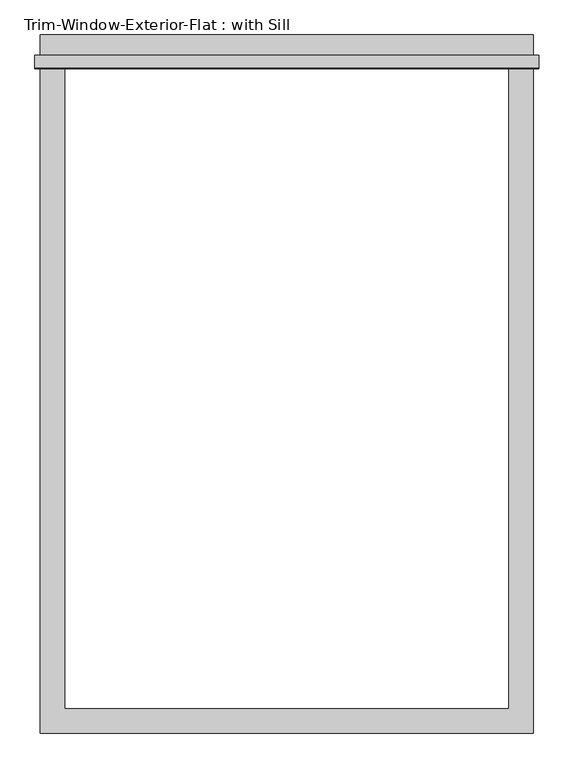
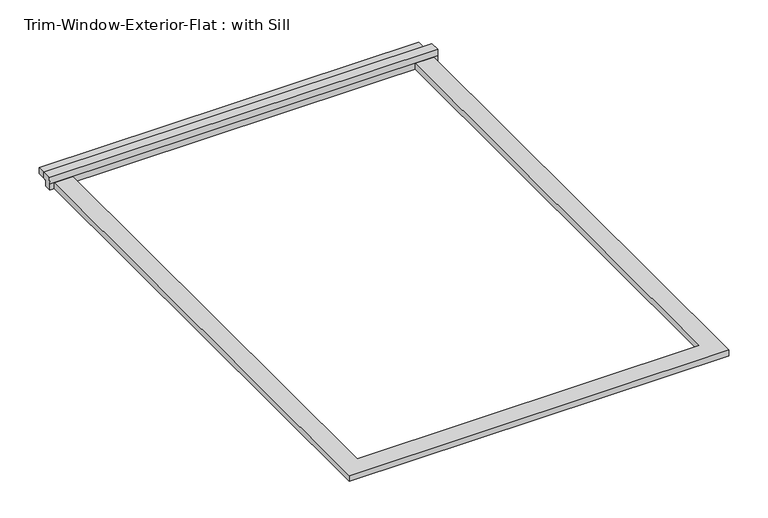
"""IFC4 building model written with IfcOpenShell, lengths in millimetres: proxy geometry, Trim-Window-Exterior-Flat : with Sill."""

from ifc_helpers import new_model, si_unit, frame, origin, origin_with_axes, place, context, project, spatial, polyline, outline, extrude, source, transform, mapped, element, save


def trim_window_exterior_flat_with_sill_a73e42ff(model_context):
    return source(origin(), model_context, "Body", "SweptSolid", [
        extrude(outline(polyline([(577.85, 1520.7823709), (-577.85, 1520.7823709), (-577.85, 1577.9323709), (577.85, 1577.9323709), (577.85, 1520.7823709)])), origin_with_axes(), (0.0, 0.0, 1.0), 19.05),
        extrude(outline(polyline([(1530.35, 38.1), (1530.35, 19.05), (1520.7823709, 19.05), (1520.7823709, 0.0), (1498.6, 0.0), (1498.6, 19.05), (1501.0580645, 38.1), (1530.35, 38.1)])), frame((-590.55, 0.0, 0.0), z_axis=(1.0, 0.0, 0.0), x_axis=(0.0, 1.0, 0.0)), (0.0, 0.0, 1.0), 1181.1),
        extrude(outline(polyline([(-577.85, -57.15), (-577.85, 1498.6), (-520.7, 1498.6), (-520.7, 0.0), (520.7, 0.0), (520.7, 1498.6), (577.85, 1498.6), (577.85, -57.15), (-577.85, -57.15)])), origin_with_axes(), (0.0, 0.0, 1.0), 19.05),
    ])


if __name__ == "__main__":
    model = new_model("IFC4")
    model_context = context("Model", 3, world=origin())
    ifc_project = project(units=[si_unit("LENGTHUNIT", "METRE", prefix="MILLI")], contexts=[model_context])
    site = spatial("IfcSite", under=ifc_project)
    building = spatial("IfcBuilding", under=site)
    placement = place(None, origin())
    trim_window_exterior_flat_with_sill_shape = trim_window_exterior_flat_with_sill_a73e42ff(model_context)
    element("IfcBuildingElementProxy", 1, Name="Trim-Window-Exterior-Flat : with Sill", ObjectType="Trim-Window-Exterior-Flat : with Sill", at=placement, inside=building, context=model_context, shape_type="MappedRepresentation", body=[
        mapped(trim_window_exterior_flat_with_sill_shape, transform((0.0, 0.0, 0.0), x_axis=(1.0, 0.0, 0.0), y_axis=(0.0, 1.0, 0.0), z_axis=(0.0, 0.0, 1.0))),
    ])
    save(model, "model.ifc")

# Revit data of these elements
# Type "Trim-Window-Exterior-Flat : with Sill"
#   Trim Width = 0' - 2 1/4"
#   Trim Thickness_Picture Frame = 0' - 1 1/4"
#   Trim Thickness_with Sill = 0' - 0 3/4"
#   Sill Thickness = 0' - 1 1/4"
#   Opening Width [instance default] = 2' - 0"
#   Opening Height [instance default] = 3' - 0"
#   Default Elevation = 4' - 0"
#   Sill = yes
#   Picture Frame = no
#   Trim Material [instance default] = none
# Element 1 (IfcBuildingElementProxy, "Trim-Window-Exterior-Flat : with Sill")
#   Opening Width = 3' - 5"
#   Opening Height = 4' - 11"
#   Trim Material = Clad - White
#   Materials on its faces: "Clad - White"
# Materials
#   "Clad - White": class "Wood", colour RGB 242 242 238, transparency 0, Cost = 0
